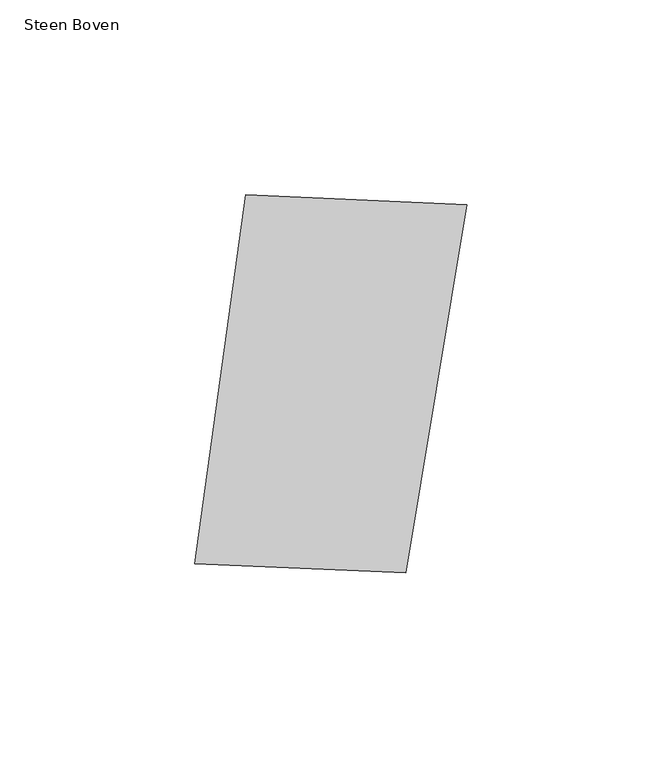
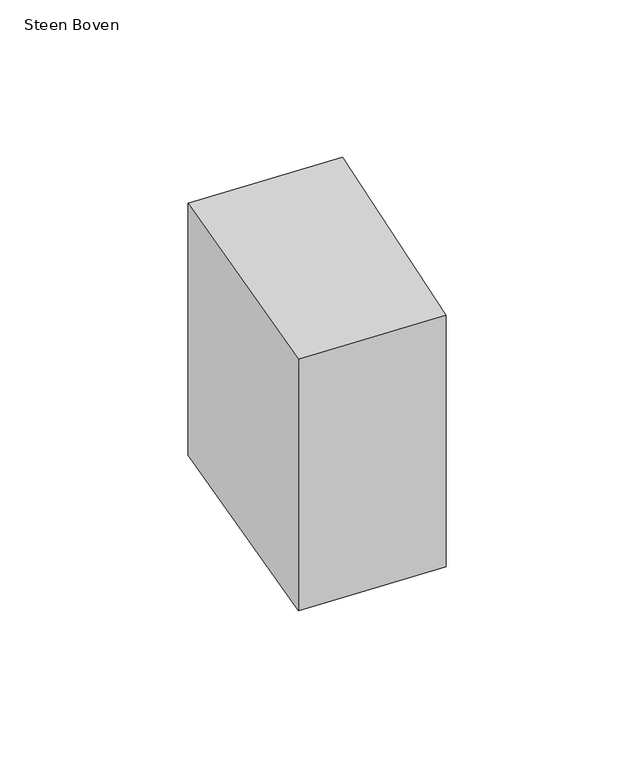
"""IFC4 building model written with IfcOpenShell, lengths in millimetres: proxy geometry, 00_GMA_steen_versie_4 : Steen Boven."""

from ifc_helpers import new_model, si_unit, origin, origin_with_axes, place, context, project, spatial, polyline, outline, extrude, source, transform, mapped, element, save


def steen_boven_0816abee(model_context):
    return source(origin(), model_context, "Body", "SweptSolid", [
        extrude(outline(polyline([(108.7495774, 118.5040405), (93.1797198, 24.0625342), (39.1014603, 26.4532894), (52.1376616, 120.9944422), (108.7495774, 118.5040405)])), origin_with_axes(), (0.0, 0.0, 1.0), 100.0),
    ])


if __name__ == "__main__":
    model = new_model("IFC4")
    model_context = context("Model", 3, world=origin())
    ifc_project = project(units=[si_unit("LENGTHUNIT", "METRE", prefix="MILLI")], contexts=[model_context])
    site = spatial("IfcSite", under=ifc_project)
    building = spatial("IfcBuilding", under=site)
    placement = place(None, origin())
    steen_boven_shape = steen_boven_0816abee(model_context)
    element("IfcBuildingElementProxy", 1, Name="00_GMA_steen_versie_4 : Steen Boven", ObjectType="00_GMA_steen_versie_4 : Steen Boven", at=placement, inside=building, context=model_context, shape_type="MappedRepresentation", body=[
        mapped(steen_boven_shape, transform((0.0, 0.0, 0.0), x_axis=(1.0, 0.0, 0.0), y_axis=(0.0, 1.0, 0.0), z_axis=(0.0, 0.0, 1.0))),
    ])
    save(model, "model.ifc")

# Revit data of these elements
# Type "00_GMA_steen_versie_4 : Steen Boven"
#   StootVoegHalfBoven [instance default] = 5 mm
#   StootVoegHalf [instance default] = 5 mm
#   StootVoegBreedteOnder = 10 mm
#   StootVoegBreedteBoven = 10 mm
#   Steendikte = 100 mm
#   LintVoegOnderHalf = 5 mm
#   LintVoegOnder = 10 mm
#   LintVoegBovenHalf = 0 mm
#   LintVoegBoven = 0 mm
#   materiaal = none
#   MateriaalVoeg = none
#   Default Elevation = 0
